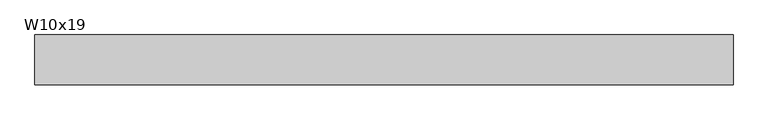
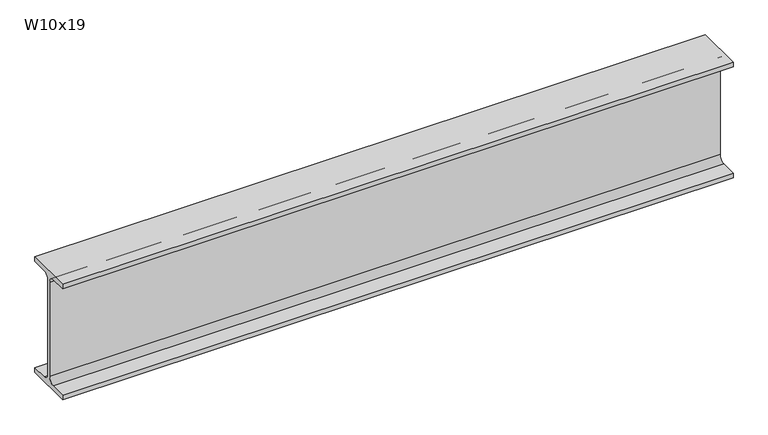
"""IFC4 building model written with IfcOpenShell, lengths in millimetres: beam geometry, RME W-Wide Flange : W10x19."""

from ifc_helpers import new_model, si_unit, point, frame, frame_2d, origin, place, context, project, spatial, polyline, circle_curve, trimmed, segment, composite_curve, outline, extrude, source, transform, mapped, element, save


def w10x19_ad57da5a(model_context):
    return source(origin(), model_context, "Body", "SweptSolid", [
        extrude(outline(composite_curve([segment(polyline([(51.054, -119.507), (51.054, -129.54), (-51.054, -129.54), (-51.054, -119.507), (-16.9545, -119.507)]), True, "CONTINUOUS"), segment(trimmed(circle_curve(frame_2d((-16.9545, -105.7275)), 13.7795), [point((-16.9545, -119.507))], [point((-3.175, -105.7275))], True, "CARTESIAN"), True, "CONTINUOUS"), segment(polyline([(-3.175, -105.7275), (-3.175, 105.7275)]), True, "CONTINUOUS"), segment(trimmed(circle_curve(frame_2d((-16.9545, 105.7275)), 13.7795), [point((-3.175, 105.7275))], [point((-16.9545, 119.507))], True, "CARTESIAN"), True, "CONTINUOUS"), segment(polyline([(-16.9545, 119.507), (-51.054, 119.507), (-51.054, 129.54), (51.054, 129.54), (51.054, 119.507), (16.9545, 119.507)]), True, "CONTINUOUS"), segment(trimmed(circle_curve(frame_2d((16.9545, 105.7275)), 13.7795), [point((16.9545, 119.507))], [point((3.175, 105.7275))], True, "CARTESIAN"), True, "CONTINUOUS"), segment(polyline([(3.175, 105.7275), (3.175, -105.7275)]), True, "CONTINUOUS"), segment(trimmed(circle_curve(frame_2d((16.9545, -105.7275)), 13.7795), [point((3.175, -105.7275))], [point((16.9545, -119.507))], True, "CARTESIAN"), True, "CONTINUOUS"), segment(polyline([(16.9545, -119.507), (51.054, -119.507)]), True, "CONTINUOUS")], self_intersect=False)), frame((-713.300409, 0.0, 0.0), z_axis=(1.0, 0.0, 0.0), x_axis=(0.0, 1.0, 0.0)), (0.0, 0.0, 1.0), 1426.600818),
    ])


if __name__ == "__main__":
    model = new_model("IFC4")
    model_context = context("Model", 3, world=origin())
    ifc_project = project(units=[si_unit("LENGTHUNIT", "METRE", prefix="MILLI")], contexts=[model_context])
    site = spatial("IfcSite", under=ifc_project)
    building = spatial("IfcBuilding", under=site)
    placement = place(None, origin())
    w10x19_shape = w10x19_ad57da5a(model_context)
    element("IfcBeam", 1, ObjectType="RME W-Wide Flange : W10x19", at=placement, inside=building, context=model_context, shape_type="MappedRepresentation", body=[
        mapped(w10x19_shape, transform((0.0, 0.0, 0.0), x_axis=(1.0, 0.0, 0.0), y_axis=(0.0, 1.0, 0.0), z_axis=(0.0, 0.0, 1.0))),
    ])
    save(model, "model.ifc")

# Revit data of these elements
# Type "RME W-Wide Flange : W10x19"
#   WELD P [instance default] = ""
#   WELD LE [instance default] = ""
#   WELD D [instance default] = ""
#   TOP SECTION SIZE [instance default] = ""
#   TOP SECTION LENGTH [instance default] = ""
#   REMARKS [instance default] = ""
#   REINF TYPE [instance default] = ""
#   Nominal Size = "W24"
#   End Bearing Capacity [instance default] = ""
#   BOT SECTION SIZE [instance default] = ""
#   BOT SECTION LENGTH [instance default] = ""
#   Assembly Code = "B10"
#   W = 19
#   Start Extension Calculation [instance default] = 10' - 0"
#   Start Extension [instance default] = -0' - 0 1/2"
#   End Extension Calculation [instance default] = 10' - 0"
#   End Extension [instance default] = -0' - 0 1/2"
#   Length [instance default] = 5' - 0"
#   bf = 0' - 4.02"
#   d = 0' - 10.2"
#   k = 0' - 0 15/16"
#   k2 = 0' - 0.5425"
#   tf = 0' - 0.395"
#   tw = 0' - 0 1/4"
#   A = 0.0390278 SF
#   Structural Material [instance default] = Metal - Steel - ASTM A992
# Element 1 (IfcBeam, "RME W-Wide Flange : W10x19")
#   Length = 4' - 8.16539"
#   Materials on its faces: "Metal - Steel - ASTM A992"
# Materials
#   "Metal - Steel - ASTM A992": class "Metal", colour RGB 255 128 0, transparency 0
